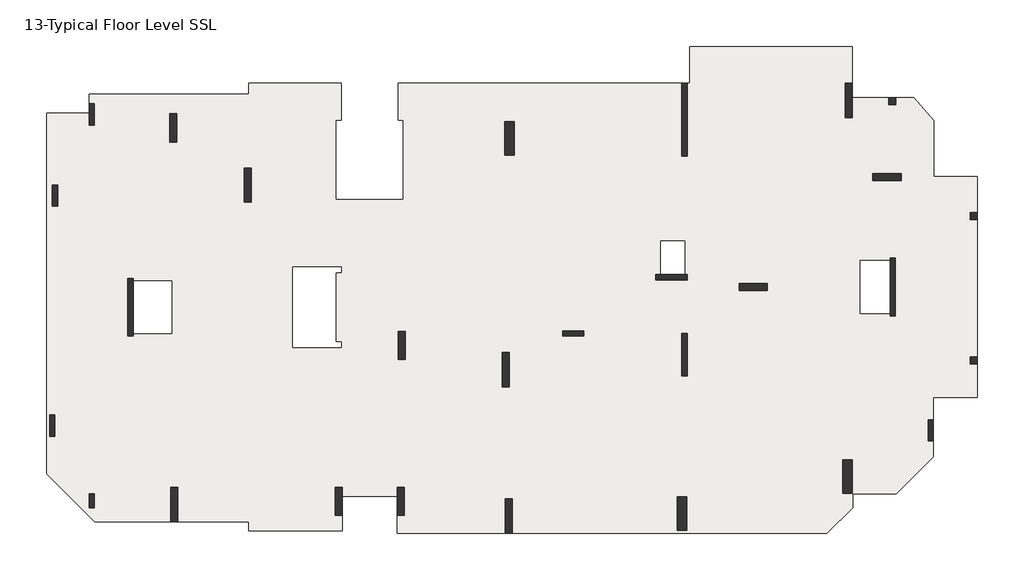
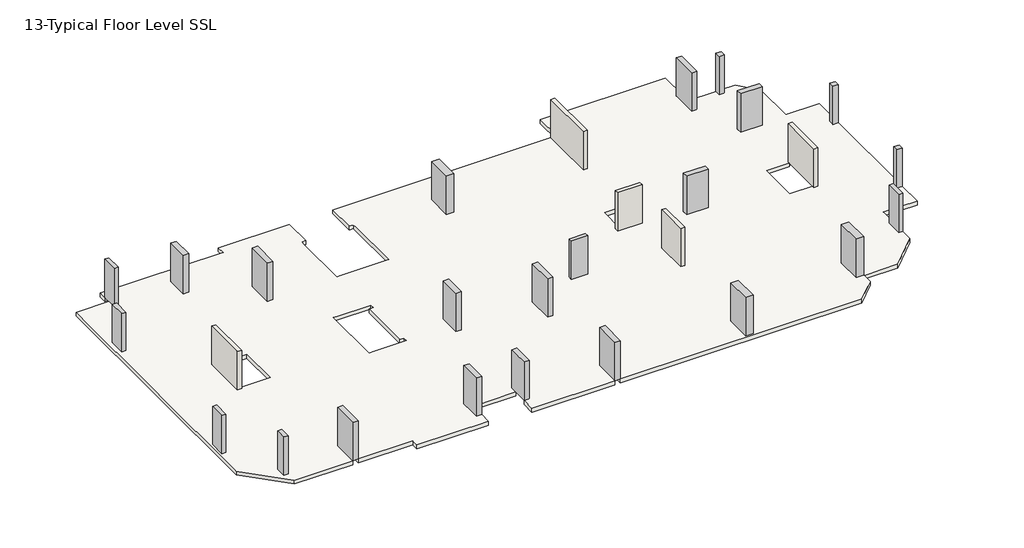
# One storey: 23 columns, 5 walls, 1 slab.
"""IFC4 building model written with IfcOpenShell, lengths in millimetres."""

import ifcopenshell
import ifcopenshell.guid

model = None  # the IFC model being written
_history = None  # IfcOwnerHistory: only IFC2X3 demands one
_inside = {}  # id of a spatial element -> (the spatial element, [elements in it])
_under = {}  # id of a project, library or spatial element -> (it, [spatial elements below it])
_declared = {}  # id of a project -> (the project, [libraries it declares])
_typed = {}  # id of a type object -> (the type object, [elements of that type])
_made_of = {}  # id of a material, layer set ... -> (it, [elements and type objects made of it])


def new_model(schema):
    """Start an empty IFC model of exactly this schema.

    Asked for "IFC4X3", IfcOpenShell would pick the latest addendum, in which some entities
    have other attributes; the version numbers below select the first issue.
    IFC2X3 requires an IfcOwnerHistory on every rooted entity: one is made here for all.
    """
    global model, _history
    if schema == "IFC4X3":
        model = ifcopenshell.file(schema_version=(4, 3, 0, 0))
    else:
        model = ifcopenshell.file(schema=schema)
    _inside.clear()
    _under.clear()
    _declared.clear()
    _typed.clear()
    _made_of.clear()
    _history = None
    if model.schema == "IFC2X3":
        org = make("IfcOrganization", Name="unknown")
        user = make(
            "IfcPersonAndOrganization",
            ThePerson=make("IfcPerson", FamilyName="unknown"),
            TheOrganization=org,
        )
        app = make(
            "IfcApplication",
            ApplicationDeveloper=org,
            Version="unknown",
            ApplicationFullName="unknown",
            ApplicationIdentifier="unknown",
        )
        _history = make(
            "IfcOwnerHistory",
            OwningUser=user,
            OwningApplication=app,
            ChangeAction="ADDED",
            CreationDate=0,
        )
    return model


def make(cls, **values):
    """One entity of the class cls with the attributes given. An attribute that is None is left unset."""
    return model.create_entity(
        cls, **{name: value for name, value in values.items() if value is not None}
    )


def rooted(cls, **values):
    """An entity with a GlobalId (a new one), such as an element, a storey or a relation."""
    return make(cls, GlobalId=ifcopenshell.guid.new(), OwnerHistory=_history, **values)


def si_unit(unit_type, name, prefix=None):
    """IfcSIUnit, for example si_unit("LENGTHUNIT", "METRE", prefix="MILLI")."""
    return make("IfcSIUnit", UnitType=unit_type, Prefix=prefix, Name=name)


def assignment(units):
    """IfcUnitAssignment: the units of a project."""
    return None if units is None else make("IfcUnitAssignment", Units=units)


def point(xyz):
    """IfcCartesianPoint."""
    return None if xyz is None else make("IfcCartesianPoint", Coordinates=xyz)


def direction(xyz):
    """IfcDirection."""
    return None if xyz is None else make("IfcDirection", DirectionRatios=xyz)


def frame(location, z_axis=None, x_axis=None):
    """IfcAxis2Placement3D, a coordinate frame: its origin and axes. An axis left out is left unset."""
    return make(
        "IfcAxis2Placement3D",
        Location=point(location),
        Axis=direction(z_axis),
        RefDirection=direction(x_axis),
    )


def origin():
    """The frame at (0, 0, 0) with its axes left unset."""
    return frame((0.0, 0.0, 0.0))


def place(relative_to, where):
    """IfcLocalPlacement: puts the frame where relative to a parent placement (None: the world)."""
    return make(
        "IfcLocalPlacement", PlacementRelTo=relative_to, RelativePlacement=where
    )


def context(
    kind, dimensions, precision=None, world=None, true_north=None, identifier=None
):
    """IfcGeometricRepresentationContext, for example the 3D "Model" context."""
    return make(
        "IfcGeometricRepresentationContext",
        ContextIdentifier=identifier,
        ContextType=kind,
        CoordinateSpaceDimension=dimensions,
        Precision=precision,
        WorldCoordinateSystem=world,
        TrueNorth=true_north,
    )


def project(units=None, contexts=None):
    """IfcProject with its units and contexts."""
    return rooted(
        "IfcProject",
        Name="project",
        RepresentationContexts=contexts,
        UnitsInContext=assignment(units),
    )


def spatial(cls, under=None, at=None, **own):
    """A site, building, storey or space (cls), placed at a placement, below another one or the project."""
    s = rooted(cls, ObjectPlacement=at, **own)
    if under is not None:
        _under.setdefault(under.id(), (under, []))[1].append(s)
    return s


def faces_of(points, faces, orient=None, outer=None):
    """IfcFace entities. A face is a list of loops; a loop is a list of indices into points, from 0.

    orient and outer hold one flag for each loop. By default every Orientation is true, the
    first loop of a face is its IfcFaceOuterBound and the others are IfcFaceBound.
    """
    made = []
    for i, loops in enumerate(faces):
        bounds = []
        for j, loop in enumerate(loops):
            is_outer = j == 0 if outer is None else outer[i][j]
            bounds.append(
                make(
                    "IfcFaceOuterBound" if is_outer else "IfcFaceBound",
                    Bound=make("IfcPolyLoop", Polygon=[points[k] for k in loop]),
                    Orientation=True if orient is None else orient[i][j],
                )
            )
        made.append(make("IfcFace", Bounds=bounds))
    return made


def faceted_brep(points, faces, orient=None, outer=None, voids=None):
    """IfcFacetedBrep: a solid bounded by flat faces; with voids (closed shells), ...WithVoids."""
    shared = [point(p) for p in points]
    hull = make("IfcClosedShell", CfsFaces=faces_of(shared, faces, orient, outer))
    if voids is None:
        return make("IfcFacetedBrep", Outer=hull)
    return make(
        "IfcFacetedBrepWithVoids",
        Outer=hull,
        Voids=[
            make(cls, CfsFaces=faces_of(shared, fs, o, b)) for cls, fs, o, b in voids
        ],
    )


def shape(context_of_items, identifier, shape_type, items):
    """IfcShapeRepresentation: the items that make up one representation, for example the "Body"."""
    return make(
        "IfcShapeRepresentation",
        ContextOfItems=context_of_items,
        RepresentationIdentifier=identifier,
        RepresentationType=shape_type,
        Items=items,
    )


def made_of(thing, what):
    """Note that an element or type object is made of a material, layer set ...; save() writes the relation."""
    if what is not None:
        _made_of.setdefault(what.id(), (what, []))[1].append(thing)
    return thing


def element(
    cls,
    number,
    at=None,
    inside=None,
    cuts=None,
    type_object=None,
    material=None,
    context=None,
    identifier="Body",
    shape_type=None,
    held_by="IfcProductDefinitionShape",
    body=None,
    shapes=None,
    **own,
):
    """One element of the class cls, such as IfcWall. Its Tag is "e" and its number.

    at: its placement. inside: the storey or other place that contains it. cuts: it is an
    opening in that element (IfcRelVoidsElement). A single representation is given by context,
    identifier, shape_type and body (its items); several are given by shapes. held_by: the class
    of the entity that holds the representations. save() writes the other relations.
    """
    e = rooted(cls, Tag="e%d" % number, ObjectPlacement=at, **own)
    if body is not None:
        shapes = [shape(context, identifier, shape_type, body)]
    if shapes is not None:
        e.Representation = make(held_by, Representations=shapes)
    if inside is not None:
        _inside.setdefault(inside.id(), (inside, []))[1].append(e)
    if cuts is not None:
        rooted(
            "IfcRelVoidsElement", RelatingBuildingElement=cuts, RelatedOpeningElement=e
        )
    if type_object is not None:
        _typed.setdefault(type_object.id(), (type_object, []))[1].append(e)
    return made_of(e, material)


def aggregate(whole, parts):
    """IfcRelAggregates: a whole, such as a stair, and the parts it consists of."""
    return rooted("IfcRelAggregates", RelatingObject=whole, RelatedObjects=parts)


def save(model, path):
    """Write the relations noted so far, then the file.

    IfcRelAggregates (storeys below a building ...), IfcRelContainedInSpatialStructure (elements
    in a storey), IfcRelDefinesByType, IfcRelAssociatesMaterial and IfcRelDeclares: one each for
    every whole, place, type object, material and project.
    """
    for whole, parts in _under.values():
        aggregate(whole, parts)
    for where, things in _inside.values():
        rooted(
            "IfcRelContainedInSpatialStructure",
            RelatedElements=things,
            RelatingStructure=where,
        )
    for kind, things in _typed.values():
        rooted("IfcRelDefinesByType", RelatedObjects=things, RelatingType=kind)
    for what, things in _made_of.values():
        rooted("IfcRelAssociatesMaterial", RelatedObjects=things, RelatingMaterial=what)
    for by, libraries in _declared.values():
        rooted("IfcRelDeclares", RelatingContext=by, RelatedDefinitions=libraries)
    model.write(path)


model = new_model("IFC4")

# Units and contexts
model_context = context("Model", 3, world=origin())
ifc_project = project(units=[si_unit("LENGTHUNIT", "METRE", prefix="MILLI")], contexts=[model_context])

# Site, building, storey
site = spatial("IfcSite", under=ifc_project)
building = spatial("IfcBuilding", under=site)
storey = spatial("IfcBuildingStorey", under=building, Name="13-Typical Floor Level SSL", Elevation=33000.0)

# Columns
placement = place(None, origin())
element("IfcColumn", 1, ObjectType="M_Concrete-Rectangular-Column : C-1 (400 x 400mm)", at=placement, inside=storey, context=model_context, shape_type="Brep", body=[
    faceted_brep([(52549.9999998, 16712.0, 33000.0), (52549.9999998, 16312.0, 33000.0), (52149.9999998, 16312.0, 33000.0), (52149.9999998, 16712.0, 33000.0), (52549.9999998, 16712.0, 36000.0), (52549.9999998, 16312.0, 36000.0), (52549.9999998, 16312.0, 35700.0), (52549.9999998, 16712.0, 35700.0), (52149.9999998, 16312.0, 36000.0), (52149.9999998, 16312.0, 35700.0), (52149.9999998, 16712.0, 36000.0), (52149.9999998, 16712.0, 35700.0)], [[[0, 1, 2, 3]], [[4, 5, 6, 1, 0, 7]], [[5, 8, 9, 2, 1, 6]], [[8, 10, 11, 3, 2, 9]], [[10, 4, 7, 0, 3, 11]], [[4, 10, 8, 5]]]),
])
element("IfcColumn", 2, ObjectType="M_Concrete-Rectangular-Column : C-1 (400 x 400mm)", at=placement, inside=storey, context=model_context, shape_type="Brep", body=[
    faceted_brep([(47898.6337868, 23252.0, 33000.0), (47898.6337868, 22852.0, 33000.0), (47498.6337868, 22852.0, 33000.0), (47498.6337868, 23252.0, 33000.0), (47898.6337868, 23252.0, 36000.0), (47898.6337868, 22852.0, 36000.0), (47898.6337868, 22852.0, 35700.0), (47498.6337868, 22852.0, 36000.0), (47498.6337868, 22852.0, 35700.0), (47498.6337868, 23252.0, 36000.0)], [[[0, 1, 2, 3]], [[4, 5, 6, 1, 0]], [[5, 7, 8, 2, 1, 6]], [[7, 9, 3, 2, 8]], [[9, 4, 0, 3]], [[4, 9, 7, 5]]]),
])
element("IfcColumn", 3, ObjectType="M_Concrete-Rectangular-Column : C-1 (400 x 400mm)", at=placement, inside=storey, context=model_context, shape_type="Brep", body=[
    faceted_brep([(52549.9999998, 8504.0039609, 33000.0), (52549.9999998, 8104.0039609, 33000.0), (52149.9999998, 8104.0039609, 33000.0), (52149.9999998, 8504.0039609, 33000.0), (52549.9999998, 8504.0039609, 36000.0), (52549.9999998, 8104.0039609, 36000.0), (52549.9999998, 8104.0039609, 35700.0), (52549.9999998, 8504.0039609, 35700.0), (52149.9999998, 8104.0039609, 36000.0), (52149.9999998, 8104.0039609, 35700.0), (52149.9999998, 8504.0039609, 36000.0), (52149.9999998, 8504.0039609, 35700.0)], [[[0, 1, 2, 3]], [[4, 5, 6, 1, 0, 7]], [[5, 8, 9, 2, 1, 6]], [[8, 10, 11, 3, 2, 9]], [[10, 4, 7, 0, 3, 11]], [[4, 10, 8, 5]]]),
])
element("IfcColumn", 4, ObjectType="M_Concrete-Rectangular-Column : C-2 (300 x 800mm)", at=placement, inside=storey, context=model_context, shape_type="Brep", body=[
    faceted_brep([(2352.0, 728.0, 33000.0), (2352.0, -72.0, 33000.0), (2052.0, -72.0, 33000.0), (2052.0, 728.0, 33000.0), (2352.0, 728.0, 36000.0), (2352.0, -72.0, 36000.0), (2352.0, -72.0, 35700.0), (2352.0, 728.0, 35700.0), (2052.0, -72.0, 36000.0), (2052.0, -72.0, 35700.0), (2052.0, 728.0, 36000.0), (2052.0, 728.0, 35700.0)], [[[0, 1, 2, 3]], [[4, 5, 6, 1, 0, 7]], [[5, 8, 9, 2, 1, 6]], [[8, 10, 11, 3, 2, 9]], [[10, 4, 7, 0, 3, 11]], [[4, 10, 8, 5]]]),
])
element("IfcColumn", 5, ObjectType="M_Concrete-Rectangular-Column : C-3(300 x 1200mm)", at=placement, inside=storey, context=model_context, shape_type="Brep", body=[
    faceted_brep([(2352.0, 22908.0000656, 33000.0), (2352.0, 21708.0000656, 33000.0), (2052.0, 21708.0000656, 33000.0), (2052.0, 22908.0000656, 33000.0), (2352.0, 22908.0000656, 36000.0), (2352.0, 21708.0000656, 36000.0), (2352.0, 21708.0000656, 35700.0), (2352.0, 22908.0000656, 35700.0), (2052.0, 21708.0000656, 36000.0), (2052.0, 21708.0000656, 35700.0), (2052.0, 22380.0004589, 36000.0), (2052.0, 22908.0000656, 36000.0), (2052.0, 22908.0000656, 35700.0)], [[[0, 1, 2, 3]], [[4, 5, 6, 1, 0, 7]], [[5, 8, 9, 2, 1, 6]], [[8, 10, 11, 12, 3, 2, 9]], [[11, 4, 7, 0, 3, 12]], [[4, 11, 10, 8, 5]]]),
])
element("IfcColumn", 6, ObjectType="M_Concrete-Rectangular-Column : C-3(300 x 1200mm)", at=placement, inside=storey, context=model_context, shape_type="Brep", body=[
    faceted_brep([(257.9999999, 18288.0, 33000.0), (257.9999999, 17088.0, 33000.0), (-42.0000001, 17088.0, 33000.0), (-42.0000001, 18288.0, 33000.0), (257.9999999, 18288.0, 36000.0), (257.9999999, 17088.0, 36000.0), (257.9999999, 17088.0, 35700.0), (257.9999999, 18288.0, 35700.0), (-42.0000001, 17088.0, 36000.0), (-42.0000001, 17088.0, 35700.0), (-42.0000001, 18288.0, 36000.0), (-42.0000001, 18288.0, 35700.0)], [[[0, 1, 2, 3]], [[4, 5, 6, 1, 0, 7]], [[5, 8, 9, 2, 1, 6]], [[8, 10, 11, 3, 2, 9]], [[10, 4, 7, 0, 3, 11]], [[4, 10, 8, 5]]]),
])
element("IfcColumn", 7, ObjectType="M_Concrete-Rectangular-Column : C-3(300 x 1200mm)", at=placement, inside=storey, context=model_context, shape_type="Brep", body=[
    faceted_brep([(108.001803, 5201.9999858, 33000.0), (108.001803, 4001.9999858, 33000.0), (-191.998197, 4001.9999858, 33000.0), (-191.998197, 5201.9999858, 33000.0), (108.001803, 5201.9999858, 36000.0), (108.001803, 4001.9999858, 36000.0), (108.001803, 4001.9999858, 35700.0), (108.001803, 5201.9999858, 35700.0), (-191.998197, 4001.9999858, 36000.0), (-191.998197, 4001.9999858, 35700.0), (-191.998197, 5201.9999858, 36000.0), (-191.998197, 5201.9999858, 35700.0)], [[[0, 1, 2, 3]], [[4, 5, 6, 1, 0, 7]], [[5, 8, 9, 2, 1, 6]], [[8, 10, 11, 3, 2, 9]], [[10, 4, 7, 0, 3, 11]], [[4, 10, 8, 5]]]),
])
element("IfcColumn", 8, ObjectType="M_Concrete-Rectangular-Column : C-3(300 x 1200mm)", at=placement, inside=storey, context=model_context, shape_type="Brep", body=[
    faceted_brep([(50046.0009271, 4931.9999929, 33000.0), (50046.0009271, 3731.9999929, 33000.0), (49746.0009271, 3731.9999929, 33000.0), (49746.0009271, 4931.9999929, 33000.0), (50046.0009271, 4931.9999929, 36000.0), (50046.0009271, 3731.9999929, 36000.0), (50046.0009271, 3731.9999929, 35700.0), (50046.0009271, 4931.9999929, 35700.0), (49746.0009271, 3731.9999929, 36000.0), (49746.0009271, 3731.9999929, 35700.0), (49746.0009271, 4931.9999929, 36000.0), (49746.0009271, 4931.9999929, 35700.0)], [[[0, 1, 2, 3]], [[4, 5, 6, 1, 0, 7]], [[5, 8, 9, 2, 1, 6]], [[8, 10, 11, 3, 2, 9]], [[10, 4, 7, 0, 3, 11]], [[4, 10, 8, 5]]]),
])
element("IfcColumn", 9, ObjectType="M_Concrete-Rectangular-Column : C-3(300 x 1200mm)", at=placement, inside=storey, context=model_context, shape_type="Brep", body=[
    faceted_brep([(28975.9999998, 9996.0000019, 33000.0), (30175.9999998, 9996.0000019, 33000.0), (30175.9999998, 9696.0000019, 33000.0), (28975.9999998, 9696.0000019, 33000.0), (28975.9999998, 9996.0000019, 36000.0), (30175.9999998, 9996.0000019, 36000.0), (30175.9999998, 9996.0000019, 35700.0), (28975.9999998, 9996.0000019, 35700.0), (30175.9999998, 9696.0000019, 36000.0), (30175.9999998, 9696.0000019, 35700.0), (28975.9999998, 9696.0000019, 36000.0), (28975.9999998, 9696.0000019, 35700.0)], [[[0, 1, 2, 3]], [[4, 5, 6, 1, 0, 7]], [[5, 8, 9, 2, 1, 6]], [[8, 10, 11, 3, 2, 9]], [[10, 4, 7, 0, 3, 11]], [[4, 10, 8, 5]]]),
])
element("IfcColumn", 10, ObjectType="M_Concrete-Rectangular-Column : C-4 (400 x 1600mm)", at=placement, inside=storey, context=model_context, shape_type="Brep", body=[
    faceted_brep([(7021.9999999, 22340.0000078, 33000.0), (7021.9999999, 20740.0000078, 33000.0), (6621.9999999, 20740.0000078, 33000.0), (6621.9999999, 22340.0000078, 33000.0), (7021.9999999, 22340.0000078, 36000.0), (7021.9999999, 20740.0000078, 36000.0), (7021.9999999, 20740.0000078, 35700.0), (7021.9999999, 22340.0000078, 35700.0), (6621.9999999, 20740.0000078, 36000.0), (6621.9999999, 20740.0000078, 35700.0), (6621.9999999, 22340.0000078, 36000.0), (6621.9999999, 22340.0000078, 35700.0)], [[[0, 1, 2, 3]], [[4, 5, 6, 1, 0, 7]], [[5, 8, 9, 2, 1, 6]], [[8, 10, 11, 3, 2, 9]], [[10, 4, 7, 0, 3, 11]], [[4, 10, 8, 5]]]),
])
element("IfcColumn", 11, ObjectType="M_Concrete-Rectangular-Column : C-4 (400 x 1600mm)", at=placement, inside=storey, context=model_context, shape_type="Brep", body=[
    faceted_brep([(19969.9997488, 1087.9955348, 33000.0), (19969.9997488, -512.0044652, 33000.0), (19569.9997488, -512.0044652, 33000.0), (19569.9997488, 1087.9955348, 33000.0), (19969.9997488, 1087.9955348, 36000.0), (19969.9997488, -512.0044652, 36000.0), (19969.9997488, -512.0044652, 35700.0), (19969.9997488, 1087.9955348, 35700.0), (19569.9997488, -512.0044652, 36000.0), (19569.9997488, -512.0044652, 35700.0), (19569.9997488, 564.000519, 36000.0), (19569.9997488, 1087.9955348, 36000.0), (19569.9997488, 1087.9955348, 35700.0)], [[[0, 1, 2, 3]], [[4, 5, 6, 1, 0, 7]], [[5, 8, 9, 2, 1, 6]], [[8, 10, 11, 12, 3, 2, 9]], [[11, 4, 7, 0, 3, 12]], [[4, 11, 10, 8, 5]]]),
])
element("IfcColumn", 12, ObjectType="M_Concrete-Rectangular-Column : C-4 (400 x 1600mm)", at=placement, inside=storey, context=model_context, shape_type="Brep", body=[
    faceted_brep([(46605.9993605, 18950.0, 33000.0), (48205.9993605, 18950.0, 33000.0), (48205.9993605, 18550.0, 33000.0), (46605.9993605, 18550.0, 33000.0), (46605.9993605, 18950.0, 36000.0), (48205.9993605, 18950.0, 36000.0), (48205.9993605, 18950.0, 35700.0), (46605.9993605, 18950.0, 35700.0), (48205.9993605, 18550.0, 36000.0), (48205.9993605, 18550.0, 35700.0), (46605.9993605, 18550.0, 36000.0), (46605.9993605, 18550.0, 35700.0)], [[[0, 1, 2, 3]], [[4, 5, 6, 1, 0, 7]], [[5, 8, 9, 2, 1, 6]], [[8, 10, 11, 3, 2, 9]], [[10, 4, 7, 0, 3, 11]], [[4, 10, 8, 5]]]),
])
element("IfcColumn", 13, ObjectType="M_Concrete-Rectangular-Column : C-5 (400 x 1600mm)", at=placement, inside=storey, context=model_context, shape_type="Brep", body=[
    faceted_brep([(20030.000009, 9955.9999979, 33000.0), (20030.000009, 8355.9999979, 33000.0), (19630.000009, 8355.9999979, 33000.0), (19630.000009, 9955.9999979, 33000.0), (20030.000009, 9955.9999979, 36000.0), (20030.000009, 8355.9999979, 36000.0), (20030.000009, 8355.9999979, 35700.0), (20030.000009, 9955.9999979, 35700.0), (19630.000009, 8355.9999979, 36000.0), (19630.000009, 8355.9999979, 35700.0), (19630.000009, 9955.9999979, 36000.0), (19630.000009, 9955.9999979, 35700.0)], [[[0, 1, 2, 3]], [[4, 5, 6, 1, 0, 7]], [[5, 8, 9, 2, 1, 6]], [[8, 10, 11, 3, 2, 9]], [[10, 4, 7, 0, 3, 11]], [[4, 10, 8, 5]]]),
])
element("IfcColumn", 14, ObjectType="M_Concrete-Rectangular-Column : C-5 (400 x 1600mm)", at=placement, inside=storey, context=model_context, shape_type="Brep", body=[
    faceted_brep([(16429.9999981, 1088.0, 33000.0), (16429.9999981, -512.0, 33000.0), (16029.9999981, -512.0, 33000.0), (16029.9999981, 1088.0, 33000.0), (16429.9999981, 1088.0, 36000.0), (16429.9999981, 564.000519, 36000.0), (16429.9999981, -512.0, 36000.0), (16429.9999981, -512.0, 35700.0), (16429.9999981, 1088.0, 35700.0), (16029.9999981, -512.0, 36000.0), (16029.9999981, -512.0, 35700.0), (16029.9999981, 1088.0, 36000.0), (16029.9999981, 1088.0, 35700.0)], [[[0, 1, 2, 3]], [[4, 5, 6, 7, 1, 0, 8]], [[6, 9, 10, 2, 1, 7]], [[9, 11, 12, 3, 2, 10]], [[11, 4, 8, 0, 3, 12]], [[4, 11, 9, 6, 5]]]),
])
element("IfcColumn", 15, ObjectType="M_Concrete-Rectangular-Column : C-5 (400 x 1600mm)", at=placement, inside=storey, context=model_context, shape_type="Brep", body=[
    faceted_brep([(38998.0014887, 12692.0079212, 33000.0), (40598.0014887, 12692.0079212, 33000.0), (40598.0014887, 12292.0079212, 33000.0), (38998.0014887, 12292.0079212, 33000.0), (38998.0014887, 12692.0079212, 36000.0), (40598.0014887, 12692.0079212, 36000.0), (40598.0014887, 12692.0079212, 35700.0), (38998.0014887, 12692.0079212, 35700.0), (40598.0014887, 12292.0079212, 36000.0), (40598.0014887, 12292.0079212, 35700.0), (38998.0014887, 12292.0079212, 36000.0), (38998.0014887, 12292.0079212, 35700.0)], [[[0, 1, 2, 3]], [[4, 5, 6, 1, 0, 7]], [[5, 8, 9, 2, 1, 6]], [[8, 10, 11, 3, 2, 9]], [[10, 4, 7, 0, 3, 11]], [[4, 10, 8, 5]]]),
])
element("IfcColumn", 16, ObjectType="M_Concrete-Rectangular-Column : C-6 (400 x 1950mm)", at=placement, inside=storey, context=model_context, shape_type="Brep", body=[
    faceted_brep([(11270.0000427, 19262.9999996, 33000.0), (11270.0000427, 17312.9999996, 33000.0), (10870.0000427, 17312.9999996, 33000.0), (10870.0000427, 19262.9999996, 33000.0), (11270.0000427, 19262.9999996, 36000.0), (11270.0000427, 17312.9999996, 36000.0), (11270.0000427, 17312.9999996, 35700.0), (11270.0000427, 19262.9999996, 35700.0), (10870.0000427, 17312.9999996, 36000.0), (10870.0000427, 17312.9999996, 35700.0), (10870.0000427, 19262.9999996, 36000.0), (10870.0000427, 19262.9999996, 35700.0)], [[[0, 1, 2, 3]], [[4, 5, 6, 1, 0, 7]], [[5, 8, 9, 2, 1, 6]], [[8, 10, 11, 3, 2, 9]], [[10, 4, 7, 0, 3, 11]], [[4, 10, 8, 5]]]),
])
element("IfcColumn", 17, ObjectType="M_Concrete-Rectangular-Column : C-6 (400 x 1950mm)", at=placement, inside=storey, context=model_context, shape_type="Brep", body=[
    faceted_brep([(7082.0000416, 1083.0000153, 33000.0), (7082.0000416, -866.9999847, 33000.0), (6682.0000416, -866.9999847, 33000.0), (6682.0000416, 1083.0000153, 33000.0), (7082.0000416, 1083.0000153, 36000.0), (7082.0000416, -866.9999847, 36000.0), (7082.0000416, -866.9999847, 35700.0), (7082.0000416, 1083.0000153, 35700.0), (6682.0000416, -866.9999847, 36000.0), (6682.0000416, -866.9999847, 35700.0), (6682.0000416, 1083.0000153, 36000.0), (6682.0000416, 1083.0000153, 35700.0)], [[[0, 1, 2, 3]], [[4, 5, 6, 1, 0, 7]], [[5, 8, 9, 2, 1, 6]], [[8, 10, 11, 3, 2, 9]], [[10, 4, 7, 0, 3, 11]], [[4, 10, 8, 5]]]),
])
element("IfcColumn", 18, ObjectType="M_Concrete-Rectangular-Column : C-6 (400 x 1950mm)", at=placement, inside=storey, context=model_context, shape_type="Brep", body=[
    faceted_brep([(26113.9999998, 422.995535, 33000.0), (26113.9999998, -1527.004465, 33000.0), (25713.9999998, -1527.004465, 33000.0), (25713.9999998, 422.995535, 33000.0), (26113.9999998, 422.995535, 36000.0), (26113.9999998, -1527.004465, 36000.0), (26113.9999998, -1527.004465, 35700.0), (26113.9999998, 422.995535, 35700.0), (25713.9999998, -1527.004465, 36000.0), (25713.9999998, -1527.004465, 35700.0), (25713.9999998, 422.995535, 36000.0), (25713.9999998, 422.995535, 35700.0)], [[[0, 1, 2, 3]], [[4, 5, 6, 1, 0, 7]], [[5, 8, 9, 2, 1, 6]], [[8, 10, 11, 3, 2, 9]], [[10, 4, 7, 0, 3, 11]], [[4, 10, 8, 5]]]),
])
element("IfcColumn", 19, ObjectType="M_Concrete-Rectangular-Column : C-6 (400 x 1950mm)", at=placement, inside=storey, context=model_context, shape_type="Brep", body=[
    faceted_brep([(45446.0007483, 24087.0, 33000.0), (45446.0007483, 22137.0, 33000.0), (45046.0007483, 22137.0, 33000.0), (45046.0007483, 24087.0, 33000.0), (45446.0007483, 24087.0, 36000.0), (45446.0007483, 23252.0000315, 36000.0), (45446.0007483, 22137.0, 36000.0), (45446.0007483, 22137.0, 35700.0), (45446.0007483, 24087.0, 35700.0), (45046.0007483, 22137.0, 36000.0), (45046.0007483, 22137.0, 35700.0), (45046.0007483, 24087.0, 36000.0), (45046.0007483, 24087.0, 35700.0)], [[[0, 1, 2, 3]], [[4, 5, 6, 7, 1, 0, 8]], [[6, 9, 10, 2, 1, 7]], [[9, 11, 12, 3, 2, 10]], [[11, 4, 8, 0, 3, 12]], [[4, 11, 9, 6, 5]]]),
])
element("IfcColumn", 20, ObjectType="M_Concrete-Rectangular-Column : C-6 (400 x 1950mm)", at=placement, inside=storey, context=model_context, shape_type="Brep", body=[
    faceted_brep([(25934.0000455, 8751.0001824, 33000.0), (25934.0000455, 6801.0001824, 33000.0), (25534.0000455, 6801.0001824, 33000.0), (25534.0000455, 8751.0001824, 33000.0), (25934.0000455, 8751.0001824, 36000.0), (25934.0000455, 6801.0001824, 36000.0), (25934.0000455, 6801.0001824, 35700.0), (25934.0000455, 8751.0001824, 35700.0), (25534.0000455, 6801.0001824, 36000.0), (25534.0000455, 6801.0001824, 35700.0), (25534.0000455, 8751.0001824, 36000.0), (25534.0000455, 8751.0001824, 35700.0)], [[[0, 1, 2, 3]], [[4, 5, 6, 1, 0, 7]], [[5, 8, 9, 2, 1, 6]], [[8, 10, 11, 3, 2, 9]], [[10, 4, 7, 0, 3, 11]], [[4, 10, 8, 5]]]),
])
element("IfcColumn", 21, ObjectType="M_Concrete-Rectangular-Column : C-7 (550 x 1900mm)", at=placement, inside=storey, context=model_context, shape_type="Brep", body=[
    faceted_brep([(36035.9999998, 548.0007983, 33000.0), (36035.9999998, -1351.9992017, 33000.0), (35485.9999998, -1351.9992017, 33000.0), (35485.9999998, 548.0007983, 33000.0), (36035.9999998, 548.0007983, 36000.0), (36035.9999998, -1351.9992017, 36000.0), (36035.9999998, -1351.9992017, 35700.0), (36035.9999998, 548.0007983, 35700.0), (35485.9999998, -1351.9992017, 36000.0), (35485.9999998, -1351.9992017, 35700.0), (35485.9999998, 548.0007983, 36000.0), (35485.9999998, 548.0007983, 35700.0)], [[[0, 1, 2, 3]], [[4, 5, 6, 1, 0, 7]], [[5, 8, 9, 2, 1, 6]], [[8, 10, 11, 3, 2, 9]], [[10, 4, 7, 0, 3, 11]], [[4, 10, 8, 5]]]),
])
element("IfcColumn", 22, ObjectType="M_Concrete-Rectangular-Column : C-7 (550 x 1900mm)", at=placement, inside=storey, context=model_context, shape_type="Brep", body=[
    faceted_brep([(45443.9999998, 2648.0, 33000.0), (45443.9999998, 748.0, 33000.0), (44893.9999998, 748.0, 33000.0), (44893.9999998, 2648.0, 33000.0), (45443.9999998, 2648.0, 36000.0), (45443.9999998, 748.0, 36000.0), (45443.9999998, 748.0, 35700.0), (45443.9999998, 2648.0, 35700.0), (44893.9999998, 748.0, 36000.0), (44893.9999998, 748.0, 35700.0), (44893.9999998, 2648.0, 36000.0), (44893.9999998, 2648.0, 35700.0)], [[[0, 1, 2, 3]], [[4, 5, 6, 1, 0, 7]], [[5, 8, 9, 2, 1, 6]], [[8, 10, 11, 3, 2, 9]], [[10, 4, 7, 0, 3, 11]], [[4, 10, 8, 5]]]),
])
element("IfcColumn", 23, ObjectType="M_Concrete-Rectangular-Column : C-7 (550 x 1900mm)", at=placement, inside=storey, context=model_context, shape_type="Brep", body=[
    faceted_brep([(26218.9999998, 21900.0, 33000.0), (26218.9999998, 20000.0, 33000.0), (25668.9999998, 20000.0, 33000.0), (25668.9999998, 21900.0, 33000.0), (26218.9999998, 21900.0, 36000.0), (26218.9999998, 20000.0, 36000.0), (26218.9999998, 20000.0, 35700.0), (26218.9999998, 21900.0, 35700.0), (25668.9999998, 20000.0, 36000.0), (25668.9999998, 20000.0, 35700.0), (25668.9999998, 21900.0, 36000.0), (25668.9999998, 21900.0, 35700.0)], [[[0, 1, 2, 3]], [[4, 5, 6, 1, 0, 7]], [[5, 8, 9, 2, 1, 6]], [[8, 10, 11, 3, 2, 9]], [[10, 4, 7, 0, 3, 11]], [[4, 10, 8, 5]]]),
])

# Slab
element("IfcSlab", 24, ObjectType="Generic 300mm", at=placement, inside=storey, context=model_context, shape_type="Brep", body=[
    faceted_brep([(36192.0021644, 24072.000519, 32700.0), (36192.0021644, 26172.000519, 32700.0), (45446.0007483, 26172.000519, 32700.0), (45446.0007483, 24087.0, 32700.0), (45046.0007483, 24087.0, 32700.0), (45046.0007483, 22137.0, 32700.0), (45446.0007483, 22137.0, 32700.0), (45446.0007483, 23252.0000315, 32700.0), (47498.6337868, 23252.0000315, 32700.0), (47498.6337868, 22852.0, 32700.0), (47898.6337868, 22852.0, 32700.0), (47898.6337868, 23252.0000315, 32700.0), (48936.764334, 23252.0000315, 32700.0), (50076.0016214, 21956.8283806, 32700.0), (50076.0016214, 18780.0084406, 32700.0), (52549.9999998, 18780.0084406, 32700.0), (52549.9999998, 16712.0, 32700.0), (52149.9999998, 16712.0, 32700.0), (52149.9999998, 16312.0, 32700.0), (52549.9999998, 16312.0, 32700.0), (52549.9999998, 8504.0039609, 32700.0), (52149.9999998, 8504.0039609, 32700.0), (52149.9999998, 8104.0039609, 32700.0), (52549.9999998, 8104.0039609, 32700.0), (52549.9999998, 6204.0084406, 32700.0), (50046.0009271, 6204.0084406, 32700.0), (50046.0009271, 4931.9999929, 32700.0), (49746.0009271, 4931.9999929, 32700.0), (49746.0009271, 3731.9999929, 32700.0), (50046.0009271, 3731.9999929, 32700.0), (50046.0009271, 2810.5958657, 32700.0), (47943.4055804, 708.000519, 32700.0), (45456.0017287, 708.000519, 32700.0), (45456.0017287, -61.7051085, 32700.0), (43990.7023722, -1527.004465, 32700.0), (26113.9999998, -1527.004465, 32700.0), (26113.9999998, 422.995535, 32700.0), (25713.9999998, 422.995535, 32700.0), (25713.9999998, -1527.004465, 32700.0), (19569.9997488, -1527.004465, 32700.0), (19569.9997488, -512.0044652, 32700.0), (19969.9997488, -512.0044652, 32700.0), (19969.9997488, 1087.9955348, 32700.0), (19569.9997488, 1087.9955348, 32700.0), (19569.9997488, 564.000519, 32700.0), (16429.9999981, 564.000519, 32700.0), (16429.9999981, 1088.0, 32700.0), (16029.9999981, 1088.0, 32700.0), (16029.9999981, -512.0, 32700.0), (16429.9999981, -512.0, 32700.0), (16429.9999981, -1391.999481, 32700.0), (11136.0000923, -1391.999481, 32700.0), (11136.0000923, -866.9999847, 32700.0), (7082.0000416, -866.9999847, 32700.0), (7082.0000416, 1083.0000153, 32700.0), (6682.0000416, 1083.0000153, 32700.0), (6682.0000416, -866.9999847, 32700.0), (2364.4419097, -866.9999847, 32700.0), (-372.0, 1869.441925, 32700.0), (-372.0, 22380.0004589, 32700.0), (2052.0, 22380.0004589, 32700.0), (2052.0, 21708.0000656, 32700.0), (2352.0, 21708.0000656, 32700.0), (2352.0, 22908.0000656, 32700.0), (2052.0, 22908.0000656, 32700.0), (2052.0, 23472.000519, 32700.0), (11136.0000923, 23472.000519, 32700.0), (11136.0000923, 24072.000519, 32700.0), (16380.0000168, 24072.000519, 32700.0), (16380.0000168, 21972.0, 32700.0), (16079.9999997, 21972.0, 32700.0), (16079.9999997, 21672.0, 32700.0), (16079.9999997, 17468.0, 32700.0), (16379.9999997, 17468.0, 32700.0), (19619.9999997, 17468.0, 32700.0), (19919.9999997, 17468.0, 32700.0), (19919.9999997, 21672.0, 32700.0), (19919.9999997, 21972.0, 32700.0), (19619.9997365, 21972.0, 32700.0), (19619.9997365, 24072.000519, 32700.0), (35747.9999998, 24072.000519, 32700.0), (35747.9999998, 19932.0, 32700.0), (36047.9999998, 19932.0, 32700.0), (36047.9999998, 24072.000519, 32700.0), (16079.9999907, 9359.999998, 32700.0), (16079.9999907, 13320.0000002, 32700.0), (16380.0000168, 13320.0000002, 32700.0), (16380.0000168, 13620.0000002, 32700.0), (13919.9999907, 13620.0000002, 32700.0), (13619.9999907, 13620.0000002, 32700.0), (13619.9999907, 13320.0000002, 32700.0), (13619.9999907, 9359.999998, 32700.0), (13619.9999907, 9059.999998, 32700.0), (13919.9999907, 9059.999998, 32700.0), (16380.0000168, 9059.999998, 32700.0), (16380.0000168, 9359.999998, 32700.0), (4548.0000034, 9840.0000003, 32700.0), (6743.9999995, 9840.0000003, 32700.0), (6743.9999995, 12840.0000003, 32700.0), (4548.0000034, 12840.0000003, 32700.0), (4548.0000025, 12984.0000001, 32700.0), (4248.0000025, 12984.0000001, 32700.0), (4248.0000025, 9696.0, 32700.0), (4548.0000025, 9696.0, 32700.0), (47580.0014798, 13992.0079177, 32700.0), (45900.001729, 13992.0079177, 32700.0), (45900.001729, 10992.0079181, 32700.0), (47580.0014798, 10992.0079181, 32700.0), (47580.0014811, 10848.0079202, 32700.0), (47880.0014811, 10848.0079202, 32700.0), (47880.0014811, 14136.0000002, 32700.0), (47580.0014811, 14136.0000002, 32700.0), (35904.002157, 15108.0000083, 32700.0), (34548.0015145, 15108.0000083, 32700.0), (34548.0015145, 13199.9999992, 32700.0), (34248.0015201, 13199.9999992, 32700.0), (34248.0015201, 12899.9999992, 32700.0), (36048.0015201, 12899.9999992, 32700.0), (36048.0015201, 13199.9999992, 32700.0), (35904.002157, 13199.9999992, 32700.0), (257.9999999, 17088.0, 32700.0), (257.9999999, 18288.0, 32700.0), (-42.0000001, 18288.0, 32700.0), (-42.0000001, 17088.0, 32700.0), (108.001803, 4001.9999858, 32700.0), (108.001803, 5201.9999858, 32700.0), (-191.998197, 5201.9999858, 32700.0), (-191.998197, 4001.9999858, 32700.0), (30175.9999998, 9996.0000019, 32700.0), (28975.9999998, 9996.0000019, 32700.0), (28975.9999998, 9696.0000019, 32700.0), (30175.9999998, 9696.0000019, 32700.0), (7021.9999999, 20740.0000078, 32700.0), (7021.9999999, 22340.0000078, 32700.0), (6621.9999999, 22340.0000078, 32700.0), (6621.9999999, 20740.0000078, 32700.0), (48205.9993605, 18950.0, 32700.0), (46605.9993605, 18950.0, 32700.0), (46605.9993605, 18550.0, 32700.0), (48205.9993605, 18550.0, 32700.0), (20030.000009, 8355.9999979, 32700.0), (20030.000009, 9955.9999979, 32700.0), (19630.000009, 9955.9999979, 32700.0), (19630.000009, 8355.9999979, 32700.0), (11270.0000427, 17312.9999996, 32700.0), (11270.0000427, 19262.9999996, 32700.0), (10870.0000427, 19262.9999996, 32700.0), (10870.0000427, 17312.9999996, 32700.0), (40598.0014887, 12692.0079212, 32700.0), (38998.0014887, 12692.0079212, 32700.0), (38998.0014887, 12292.0079212, 32700.0), (40598.0014887, 12292.0079212, 32700.0), (2352.0, -72.0, 32700.0), (2352.0, 728.0, 32700.0), (2052.0, 728.0, 32700.0), (2052.0, -72.0, 32700.0), (25934.0000455, 6801.0001824, 32700.0), (25934.0000455, 8751.0001824, 32700.0), (25534.0000455, 8751.0001824, 32700.0), (25534.0000455, 6801.0001824, 32700.0), (36035.9999998, -1351.9992017, 32700.0), (36035.9999998, 548.0007983, 32700.0), (35485.9999998, 548.0007983, 32700.0), (35485.9999998, -1351.9992017, 32700.0), (45443.9999998, 748.0, 32700.0), (45443.9999998, 2648.0, 32700.0), (44893.9999998, 2648.0, 32700.0), (44893.9999998, 748.0, 32700.0), (26218.9999998, 20000.0, 32700.0), (26218.9999998, 21900.0, 32700.0), (25668.9999998, 21900.0, 32700.0), (25668.9999998, 20000.0, 32700.0), (35748.0054035, 9840.0000002, 32700.0), (35748.0054035, 7428.0000762, 32700.0), (36048.0054035, 7428.0000762, 32700.0), (36048.0054035, 9840.0000002, 32700.0), (36192.0021644, 26172.000519, 33000.0), (36192.0021644, 24072.000519, 33000.0), (36047.9999998, 24072.000519, 33000.0), (36047.9999998, 19932.0, 33000.0), (35747.9999998, 19932.0, 33000.0), (35747.9999998, 24072.000519, 33000.0), (19619.9997365, 24072.000519, 33000.0), (19619.9997365, 21972.0, 33000.0), (19919.9999997, 21972.0, 33000.0), (19919.9999997, 21672.0, 33000.0), (19919.9999997, 17468.0, 33000.0), (19619.9999997, 17468.0, 33000.0), (16379.9999997, 17468.0, 33000.0), (16079.9999997, 17468.0, 33000.0), (16079.9999997, 21672.0, 33000.0), (16079.9999997, 21972.0, 33000.0), (16380.0000168, 21972.0, 33000.0), (16380.0000168, 24072.000519, 33000.0), (11136.0000923, 24072.000519, 33000.0), (11136.0000923, 23472.000519, 33000.0), (2052.0, 23472.000519, 33000.0), (2052.0, 22908.0000656, 33000.0), (2352.0, 22908.0000656, 33000.0), (2352.0, 21708.0000656, 33000.0), (2052.0, 21708.0000656, 33000.0), (2052.0, 22380.0004589, 33000.0), (-372.0, 22380.0004589, 33000.0), (-372.0, 1869.441925, 33000.0), (2364.4419097, -866.9999847, 33000.0), (6682.0000416, -866.9999847, 33000.0), (6682.0000416, 1083.0000153, 33000.0), (7082.0000416, 1083.0000153, 33000.0), (7082.0000416, -866.9999847, 33000.0), (11136.0000923, -866.9999847, 33000.0), (11136.0000923, -1391.999481, 33000.0), (16429.9999981, -1391.999481, 33000.0), (16429.9999981, -512.0, 33000.0), (16029.9999981, -512.0, 33000.0), (16029.9999981, 1088.0, 33000.0), (16429.9999981, 1088.0, 33000.0), (16429.9999981, 564.000519, 33000.0), (19569.9997488, 564.000519, 33000.0), (19569.9997488, 1087.9955348, 33000.0), (19969.9997488, 1087.9955348, 33000.0), (19969.9997488, -512.0044652, 33000.0), (19569.9997488, -512.0044652, 33000.0), (19569.9997488, -1527.004465, 33000.0), (25713.9999998, -1527.004465, 33000.0), (25713.9999998, 422.995535, 33000.0), (26113.9999998, 422.995535, 33000.0), (26113.9999998, -1527.004465, 33000.0), (43990.7023722, -1527.004465, 33000.0), (45456.0017287, -61.7051085, 33000.0), (45456.0017287, 708.000519, 33000.0), (47943.4055804, 708.000519, 33000.0), (50046.0009271, 2810.5958657, 33000.0), (50046.0009271, 3731.9999929, 33000.0), (49746.0009271, 3731.9999929, 33000.0), (49746.0009271, 4931.9999929, 33000.0), (50046.0009271, 4931.9999929, 33000.0), (50046.0009271, 6204.0084406, 33000.0), (52549.9999998, 6204.0084406, 33000.0), (52549.9999998, 8104.0039609, 33000.0), (52149.9999998, 8104.0039609, 33000.0), (52149.9999998, 8504.0039609, 33000.0), (52549.9999998, 8504.0039609, 33000.0), (52549.9999998, 16312.0, 33000.0), (52149.9999998, 16312.0, 33000.0), (52149.9999998, 16712.0, 33000.0), (52549.9999998, 16712.0, 33000.0), (52549.9999998, 18780.0084406, 33000.0), (50076.0016214, 18780.0084406, 33000.0), (50076.0016214, 21956.8283806, 33000.0), (48936.764334, 23252.0000315, 33000.0), (47898.6337868, 23252.0000315, 33000.0), (47898.6337868, 22852.0, 33000.0), (47498.6337868, 22852.0, 33000.0), (47498.6337868, 23252.0000315, 33000.0), (45446.0006898, 23252.0000315, 33000.0), (45446.0007483, 22137.0, 33000.0), (45046.0007483, 22137.0, 33000.0), (45046.0007483, 24087.0, 33000.0), (45446.0007483, 24087.0, 33000.0), (45446.0007483, 26172.000519, 33000.0), (16079.9999907, 13320.0000002, 33000.0), (16079.9999907, 9359.999998, 33000.0), (16380.0000168, 9359.999998, 33000.0), (16380.0000168, 9059.999998, 33000.0), (13919.9999907, 9059.999998, 33000.0), (13619.9999907, 9059.999998, 33000.0), (13619.9999907, 9359.999998, 33000.0), (13619.9999907, 13320.0000002, 33000.0), (13619.9999907, 13620.0000002, 33000.0), (13919.9999907, 13620.0000002, 33000.0), (16380.0000168, 13620.0000002, 33000.0), (16380.0000168, 13320.0000002, 33000.0), (6743.9999995, 9840.0000003, 33000.0), (4548.0000034, 9840.0000003, 33000.0), (4548.0000025, 9696.0, 33000.0), (4248.0000025, 9696.0, 33000.0), (4248.0000025, 12984.0000001, 33000.0), (4548.0000025, 12984.0000001, 33000.0), (4548.0000025, 12840.0000003, 33000.0), (6743.9999995, 12840.0000003, 33000.0), (45900.001729, 13992.0079177, 33000.0), (47580.0014798, 13992.0079177, 33000.0), (47580.0014811, 14136.0000002, 33000.0), (47880.0014811, 14136.0000002, 33000.0), (47880.0014811, 10848.0079202, 33000.0), (47580.0014811, 10848.0079202, 33000.0), (47580.0014811, 10992.0079181, 33000.0), (45900.001729, 10992.0079181, 33000.0), (34548.0015145, 15108.0000083, 33000.0), (35904.002157, 15108.0000083, 33000.0), (35904.002157, 13199.9999992, 33000.0), (36048.0015201, 13199.9999992, 33000.0), (36048.0015201, 12899.9999992, 33000.0), (34248.0015201, 12899.9999992, 33000.0), (34248.0015201, 13199.9999992, 33000.0), (34548.0015145, 13199.9999992, 33000.0), (257.9999999, 18288.0, 33000.0), (257.9999999, 17088.0, 33000.0), (-42.0000001, 17088.0, 33000.0), (-42.0000001, 18288.0, 33000.0), (108.001803, 5201.9999858, 33000.0), (108.001803, 4001.9999858, 33000.0), (-191.998197, 4001.9999858, 33000.0), (-191.998197, 5201.9999858, 33000.0), (28975.9999998, 9996.0000019, 33000.0), (30175.9999998, 9996.0000019, 33000.0), (30175.9999998, 9696.0000019, 33000.0), (28975.9999998, 9696.0000019, 33000.0), (7021.9999999, 22340.0000078, 33000.0), (7021.9999999, 20740.0000078, 33000.0), (6621.9999999, 20740.0000078, 33000.0), (6621.9999999, 22340.0000078, 33000.0), (46605.9993605, 18950.0, 33000.0), (48205.9993605, 18950.0, 33000.0), (48205.9993605, 18550.0, 33000.0), (46605.9993605, 18550.0, 33000.0), (20030.000009, 9955.9999979, 33000.0), (20030.000009, 8355.9999979, 33000.0), (19630.000009, 8355.9999979, 33000.0), (19630.000009, 9955.9999979, 33000.0), (11270.0000427, 19262.9999996, 33000.0), (11270.0000427, 17312.9999996, 33000.0), (10870.0000427, 17312.9999996, 33000.0), (10870.0000427, 19262.9999996, 33000.0), (38998.0014887, 12692.0079212, 33000.0), (40598.0014887, 12692.0079212, 33000.0), (40598.0014887, 12292.0079212, 33000.0), (38998.0014887, 12292.0079212, 33000.0), (2352.0, 728.0, 33000.0), (2352.0, -72.0, 33000.0), (2052.0, -72.0, 33000.0), (2052.0, 728.0, 33000.0), (25934.0000455, 8751.0001824, 33000.0), (25934.0000455, 6801.0001824, 33000.0), (25534.0000455, 6801.0001824, 33000.0), (25534.0000455, 8751.0001824, 33000.0), (36035.9999998, 548.0007983, 33000.0), (36035.9999998, -1351.9992017, 33000.0), (35485.9999998, -1351.9992017, 33000.0), (35485.9999998, 548.0007983, 33000.0), (45443.9999998, 2648.0, 33000.0), (45443.9999998, 748.0, 33000.0), (44893.9999998, 748.0, 33000.0), (44893.9999998, 2648.0, 33000.0), (26218.9999998, 21900.0, 33000.0), (26218.9999998, 20000.0, 33000.0), (25668.9999998, 20000.0, 33000.0), (25668.9999998, 21900.0, 33000.0), (35748.0054035, 7428.0000762, 33000.0), (35748.0054035, 9840.0000002, 33000.0), (36048.0054035, 9840.0000002, 33000.0), (36048.0054035, 7428.0000762, 33000.0)], [[[0, 1, 2, 3, 4, 5, 6, 7, 8, 9, 10, 11, 12, 13, 14, 15, 16, 17, 18, 19, 20, 21, 22, 23, 24, 25, 26, 27, 28, 29, 30, 31, 32, 33, 34, 35, 36, 37, 38, 39, 40, 41, 42, 43, 44, 45, 46, 47, 48, 49, 50, 51, 52, 53, 54, 55, 56, 57, 58, 59, 60, 61, 62, 63, 64, 65, 66, 67, 68, 69, 70, 71, 72, 73, 74, 75, 76, 77, 78, 79, 80, 81, 82, 83], [84, 85, 86, 87, 88, 89, 90, 91, 92, 93, 94, 95], [96, 97, 98, 99, 100, 101, 102, 103], [104, 105, 106, 107, 108, 109, 110, 111], [112, 113, 114, 115, 116, 117, 118, 119], [120, 121, 122, 123], [124, 125, 126, 127], [128, 129, 130, 131], [132, 133, 134, 135], [136, 137, 138, 139], [140, 141, 142, 143], [144, 145, 146, 147], [148, 149, 150, 151], [152, 153, 154, 155], [156, 157, 158, 159], [160, 161, 162, 163], [164, 165, 166, 167], [168, 169, 170, 171], [172, 173, 174, 175]], [[176, 177, 178, 179, 180, 181, 182, 183, 184, 185, 186, 187, 188, 189, 190, 191, 192, 193, 194, 195, 196, 197, 198, 199, 200, 201, 202, 203, 204, 205, 206, 207, 208, 209, 210, 211, 212, 213, 214, 215, 216, 217, 218, 219, 220, 221, 222, 223, 224, 225, 226, 227, 228, 229, 230, 231, 232, 233, 234, 235, 236, 237, 238, 239, 240, 241, 242, 243, 244, 245, 246, 247, 248, 249, 250, 251, 252, 253, 254, 255, 256, 257, 258, 259], [260, 261, 262, 263, 264, 265, 266, 267, 268, 269, 270, 271], [272, 273, 274, 275, 276, 277, 278, 279], [280, 281, 282, 283, 284, 285, 286, 287], [288, 289, 290, 291, 292, 293, 294, 295], [296, 297, 298, 299], [300, 301, 302, 303], [304, 305, 306, 307], [308, 309, 310, 311], [312, 313, 314, 315], [316, 317, 318, 319], [320, 321, 322, 323], [324, 325, 326, 327], [328, 329, 330, 331], [332, 333, 334, 335], [336, 337, 338, 339], [340, 341, 342, 343], [344, 345, 346, 347], [348, 349, 350, 351]], [[68, 193, 192, 69]], [[182, 79, 78, 183]], [[79, 182, 181, 80]], [[177, 0, 83, 178]], [[1, 0, 177, 176]], [[2, 1, 176, 259]], [[3, 2, 259, 258]], [[249, 12, 11, 250]], [[7, 254, 253, 8]], [[13, 12, 249, 248]], [[14, 13, 248, 247]], [[15, 14, 247, 246]], [[15, 246, 245, 16]], [[237, 24, 23, 238]], [[19, 242, 241, 20]], [[25, 24, 237, 236]], [[25, 236, 235, 26]], [[231, 30, 29, 232]], [[32, 31, 230, 229]], [[33, 32, 229, 228]], [[34, 33, 228, 227]], [[34, 227, 226, 35]], [[222, 39, 38, 223]], [[39, 222, 221, 40]], [[45, 44, 217, 216]], [[211, 50, 49, 212]], [[51, 50, 211, 210]], [[52, 51, 210, 209]], [[52, 209, 208, 53]], [[204, 57, 56, 205]], [[58, 57, 204, 203]], [[59, 58, 203, 202]], [[60, 59, 202, 201]], [[196, 65, 64, 197]], [[66, 65, 196, 195]], [[67, 66, 195, 194]], [[68, 67, 194, 193]], [[31, 30, 231, 230]], [[85, 84, 261, 260]], [[72, 189, 188, 187, 186, 75, 74, 73]], [[272, 97, 96, 273]], [[97, 272, 279, 98]], [[98, 279, 278, 99]], [[280, 105, 104, 281]], [[105, 280, 287, 106]], [[106, 287, 286, 107]], [[112, 289, 288, 113]], [[113, 288, 295, 114]], [[289, 112, 119, 290]], [[62, 199, 198, 63]], [[199, 62, 61, 200]], [[200, 61, 60, 201]], [[63, 198, 197, 64]], [[120, 297, 296, 121]], [[297, 120, 123, 298]], [[298, 123, 122, 299]], [[299, 122, 121, 296]], [[124, 301, 300, 125]], [[301, 124, 127, 302]], [[302, 127, 126, 303]], [[303, 126, 125, 300]], [[28, 233, 232, 29]], [[233, 28, 27, 234]], [[234, 27, 26, 235]], [[128, 305, 304, 129]], [[305, 128, 131, 306]], [[306, 131, 130, 307]], [[307, 130, 129, 304]], [[132, 309, 308, 133]], [[309, 132, 135, 310]], [[310, 135, 134, 311]], [[311, 134, 133, 308]], [[41, 220, 219, 42]], [[220, 41, 40, 221]], [[43, 218, 217, 44]], [[218, 43, 42, 219]], [[136, 313, 312, 137]], [[313, 136, 139, 314]], [[314, 139, 138, 315]], [[315, 138, 137, 312]], [[140, 317, 316, 141]], [[317, 140, 143, 318]], [[318, 143, 142, 319]], [[319, 142, 141, 316]], [[215, 46, 45, 216]], [[48, 213, 212, 49]], [[213, 48, 47, 214]], [[214, 47, 46, 215]], [[144, 321, 320, 145]], [[321, 144, 147, 322]], [[322, 147, 146, 323]], [[323, 146, 145, 320]], [[207, 54, 53, 208]], [[55, 206, 205, 56]], [[206, 55, 54, 207]], [[225, 36, 35, 226]], [[37, 224, 223, 38]], [[224, 37, 36, 225]], [[6, 255, 254, 7]], [[255, 6, 5, 256]], [[256, 5, 4, 257]], [[257, 4, 3, 258]], [[148, 325, 324, 149]], [[325, 148, 151, 326]], [[326, 151, 150, 327]], [[327, 150, 149, 324]], [[152, 329, 328, 153]], [[329, 152, 155, 330]], [[330, 155, 154, 331]], [[331, 154, 153, 328]], [[156, 333, 332, 157]], [[333, 156, 159, 334]], [[334, 159, 158, 335]], [[335, 158, 157, 332]], [[160, 337, 336, 161]], [[337, 160, 163, 338]], [[338, 163, 162, 339]], [[339, 162, 161, 336]], [[164, 341, 340, 165]], [[341, 164, 167, 342]], [[342, 167, 166, 343]], [[343, 166, 165, 340]], [[168, 345, 344, 169]], [[345, 168, 171, 346]], [[346, 171, 170, 347]], [[347, 170, 169, 344]], [[70, 191, 190, 189, 72, 71]], [[191, 70, 69, 192]], [[77, 184, 183, 78]], [[184, 77, 76, 75, 186, 185]], [[271, 86, 85, 260]], [[87, 270, 269, 268, 89, 88]], [[86, 271, 270, 87]], [[89, 268, 267, 266, 265, 92, 91, 90]], [[92, 265, 264, 263, 94, 93]], [[95, 262, 261, 84]], [[262, 95, 94, 263]], [[277, 100, 99, 278]], [[103, 274, 273, 96]], [[101, 276, 275, 102]], [[100, 277, 276, 101]], [[274, 103, 102, 275]], [[116, 293, 292, 117]], [[118, 291, 290, 119]], [[294, 115, 114, 295]], [[117, 292, 291, 118]], [[293, 116, 115, 294]], [[172, 349, 348, 173]], [[174, 351, 350, 175]], [[173, 348, 351, 174]], [[349, 172, 175, 350]], [[285, 108, 107, 286]], [[111, 282, 281, 104]], [[109, 284, 283, 110]], [[108, 285, 284, 109]], [[282, 111, 110, 283]], [[82, 179, 178, 83]], [[180, 81, 80, 181]], [[179, 82, 81, 180]], [[18, 243, 242, 19]], [[243, 18, 17, 244]], [[244, 17, 16, 245]], [[10, 251, 250, 11]], [[251, 10, 9, 252]], [[252, 9, 8, 253]], [[22, 239, 238, 23]], [[239, 22, 21, 240]], [[240, 21, 20, 241]]]),
])

# Walls
element("IfcWall", 25, ObjectType="Shear Walls 300mm", at=placement, inside=storey, context=model_context, shape_type="Brep", body=[
    faceted_brep([(4548.0000025, 9696.0, 33000.0), (4548.0000025, 12984.0000001, 33000.0), (4548.0000025, 12984.0000001, 35700.0), (4548.0000025, 12984.0000001, 36000.0), (4548.0000025, 9696.0, 36000.0), (4548.0000025, 9696.0, 35700.0), (4248.0000025, 9696.0, 33000.0), (4248.0000025, 9696.0, 35700.0), (4248.0000025, 9696.0, 36000.0), (4248.0000025, 12984.0000001, 36000.0), (4248.0000025, 12984.0000001, 35700.0), (4248.0000025, 12984.0000001, 33000.0)], [[[0, 1, 2, 3, 4, 5]], [[6, 7, 8, 9, 10, 11]], [[1, 0, 6, 11]], [[3, 2, 1, 11, 10, 9]], [[4, 3, 9, 8]], [[0, 5, 4, 8, 7, 6]]]),
])
element("IfcWall", 26, ObjectType="Shear Walls 300mm", at=placement, inside=storey, context=model_context, shape_type="Brep", body=[
    faceted_brep([(34248.0015201, 12899.9999992, 33000.0), (36048.0015201, 12899.9999992, 33000.0), (36048.0015201, 12899.9999992, 35700.0), (36048.0015201, 12899.9999992, 36000.0), (34248.0015201, 12899.9999992, 36000.0), (34248.0015201, 12899.9999992, 35700.0), (34248.0015201, 13199.9999992, 33000.0), (34248.0015201, 13199.9999992, 35700.0), (34248.0015201, 13199.9999992, 36000.0), (36048.0015201, 13199.9999992, 36000.0), (36048.0015201, 13199.9999992, 35700.0), (36048.0015201, 13199.9999992, 33000.0)], [[[0, 1, 2, 3, 4, 5]], [[6, 7, 8, 9, 10, 11]], [[1, 0, 6, 11]], [[3, 2, 1, 11, 10, 9]], [[4, 3, 9, 8]], [[0, 5, 4, 8, 7, 6]]]),
])
element("IfcWall", 27, ObjectType="Shear Walls 300mm", at=placement, inside=storey, context=model_context, shape_type="Brep", body=[
    faceted_brep([(35748.0054035, 9840.0000002, 33000.0), (35748.0054035, 7428.0000762, 33000.0), (35748.0054035, 7428.0000762, 35700.0), (35748.0054035, 7428.0000762, 36000.0), (35748.0054035, 9840.0000002, 36000.0), (35748.0054035, 9840.0000002, 35700.0), (36048.0054035, 9840.0000002, 33000.0), (36048.0054035, 9840.0000002, 35700.0), (36048.0054035, 9840.0000002, 36000.0), (36048.0054035, 7428.0000762, 36000.0), (36048.0054035, 7428.0000762, 35700.0), (36048.0054035, 7428.0000762, 33000.0)], [[[0, 1, 2, 3, 4, 5]], [[6, 7, 8, 9, 10, 11]], [[1, 0, 6, 11]], [[3, 2, 1, 11, 10, 9]], [[4, 3, 9, 8]], [[0, 5, 4, 8, 7, 6]]]),
])
element("IfcWall", 28, ObjectType="Shear Walls 300mm", at=placement, inside=storey, context=model_context, shape_type="Brep", body=[
    faceted_brep([(47580.0014811, 14136.0000002, 33000.0), (47580.0014811, 10848.0079202, 33000.0), (47580.0014811, 10848.0079202, 35700.0), (47580.0014811, 10848.0079202, 36000.0), (47580.0014811, 14136.0000002, 36000.0), (47580.0014811, 14136.0000002, 35700.0), (47880.0014811, 14136.0000002, 33000.0), (47880.0014811, 14136.0000002, 35700.0), (47880.0014811, 14136.0000002, 36000.0), (47880.0014811, 10848.0079202, 36000.0), (47880.0014811, 10848.0079202, 35700.0), (47880.0014811, 10848.0079202, 33000.0)], [[[0, 1, 2, 3, 4, 5]], [[6, 7, 8, 9, 10, 11]], [[1, 0, 6, 11]], [[3, 2, 1, 11, 10, 9]], [[4, 3, 9, 8]], [[0, 5, 4, 8, 7, 6]]]),
])
element("IfcWall", 29, ObjectType="Shear Walls 300mm", at=placement, inside=storey, context=model_context, shape_type="Brep", body=[
    faceted_brep([(36047.9999998, 19932.0, 33000.0), (36047.9999998, 24072.0078999, 33000.0), (36047.9999998, 24072.0078999, 36000.0), (36047.9999998, 19932.0, 36000.0), (36047.9999998, 19932.0, 35700.0), (35747.9999998, 19932.0, 33000.0), (35747.9999998, 19932.0, 35700.0), (35747.9999998, 19932.0, 36000.0), (35747.9999998, 24072.0078999, 36000.0), (35747.9999998, 24072.0078999, 33000.0)], [[[0, 1, 2, 3, 4]], [[5, 6, 7, 8, 9]], [[1, 0, 5, 9]], [[2, 1, 9, 8]], [[3, 2, 8, 7]], [[0, 4, 3, 7, 6, 5]]]),
])

save(model, "model.ifc")

# Revit data of these elements
# Type "M_Concrete-Rectangular-Column : C-1 (400 x 400mm)"
#   Type Mark = "C01"
#   b = 400 mm
#   h = 400 mm
#   Structural Material [instance default] = Concrete, Cast-in-Place gray
# Type "M_Concrete-Rectangular-Column : C-2 (300 x 800mm)"
#   Type Mark = "C02"
#   b = 300 mm
#   h = 800 mm
#   Structural Material [instance default] = Concrete, Cast-in-Place gray
# Type "M_Concrete-Rectangular-Column : C-3(300 x 1200mm)"
#   Type Mark = "C03"
#   b = 300 mm
#   h = 1200 mm
#   Structural Material [instance default] = Concrete, Cast-in-Place gray
# Type "M_Concrete-Rectangular-Column : C-4 (400 x 1600mm)"
#   Type Mark = "C04"
#   b = 400 mm
#   h = 1600 mm
#   Structural Material [instance default] = Concrete, Cast-in-Place gray
# Type "M_Concrete-Rectangular-Column : C-5 (400 x 1600mm)"
#   Type Mark = "C05"
#   b = 400 mm
#   h = 1600 mm
#   Structural Material [instance default] = Concrete, Cast-in-Place gray
# Type "M_Concrete-Rectangular-Column : C-6 (400 x 1950mm)"
#   Type Mark = "C06"
#   b = 400 mm
#   h = 1950 mm
#   Structural Material [instance default] = Concrete, Cast-in-Place gray
# Type "M_Concrete-Rectangular-Column : C-7 (550 x 1900mm)"
#   Type Mark = "C07"
#   b = 550 mm
#   h = 1900 mm
#   Structural Material [instance default] = Concrete, Cast-in-Place gray
# Type "Generic 300mm"
#   Function = 0
#   Layers, outside or top first: 300 mm "Concrete-RC" (function 1)
# Type "Shear Walls 300mm"
#   Layers, outside or top first: 300 mm "Concrete-RC" (function 1)
# Elements 1, 2, 3 (IfcColumn, "M_Concrete-Rectangular-Column : C-1 (400 x 400mm)")
#   Structural Material = Concrete-RC
#   Phase Created = New Construction
#   Materials on its faces: "Concrete-RC"
# Element 4 (IfcColumn, "M_Concrete-Rectangular-Column : C-2 (300 x 800mm)")
#   Structural Material = Concrete-RC
#   Phase Created = New Construction
#   Materials on its faces: "Concrete-RC"
# Elements 5, 6, 7, 8, 9 (IfcColumn, "M_Concrete-Rectangular-Column : C-3(300 x 1200mm)")
#   Structural Material = Concrete-RC
#   Phase Created = New Construction
#   Materials on its faces: "Concrete-RC"
# Elements 10, 11, 12 (IfcColumn, "M_Concrete-Rectangular-Column : C-4 (400 x 1600mm)")
#   Structural Material = Concrete-RC
#   Phase Created = New Construction
#   Materials on its faces: "Concrete-RC"
# Elements 13, 14, 15 (IfcColumn, "M_Concrete-Rectangular-Column : C-5 (400 x 1600mm)")
#   Structural Material = Concrete-RC
#   Phase Created = New Construction
#   Materials on its faces: "Concrete-RC"
# Elements 16, 17, 18, 19, 20 (IfcColumn, "M_Concrete-Rectangular-Column : C-6 (400 x 1950mm)")
#   Structural Material = Concrete-RC
#   Phase Created = New Construction
#   Materials on its faces: "Concrete-RC"
# Elements 21, 22, 23 (IfcColumn, "M_Concrete-Rectangular-Column : C-7 (550 x 1900mm)")
#   Structural Material = Concrete-RC
#   Phase Created = New Construction
#   Materials on its faces: "Concrete-RC"
# Element 24 (IfcSlab, "Generic 300mm")
#   Height Offset From Level = 0 mm
#   built-in parameter 1001954 = 1
#   Phase Created = New Construction
#   Materials on its faces: "Concrete-RC"
# Elements 25, 26, 27, 28, 29 (IfcWall, "Shear Walls 300mm")
#   Top Offset = 0 mm
#   Base Offset = 0 mm
#   wall height = 3000 mm
#   Phase Created = New Construction
#   Base Constraint = 13-Typical Floor Level SSL
#   Top Constraint = 14-Roof Level SSL
#   Materials on its faces: "Concrete-RC"
# Materials
#   "Concrete, Cast-in-Place gray": class "Concrete", colour RGB 192 192 192, transparency 0, Description = "Cast-in-place concrete", Cost = 0
#   "Concrete-RC": class "Concrete", colour RGB 128 128 128, transparency 0, Description = "High strength concrete", Cost = 0
